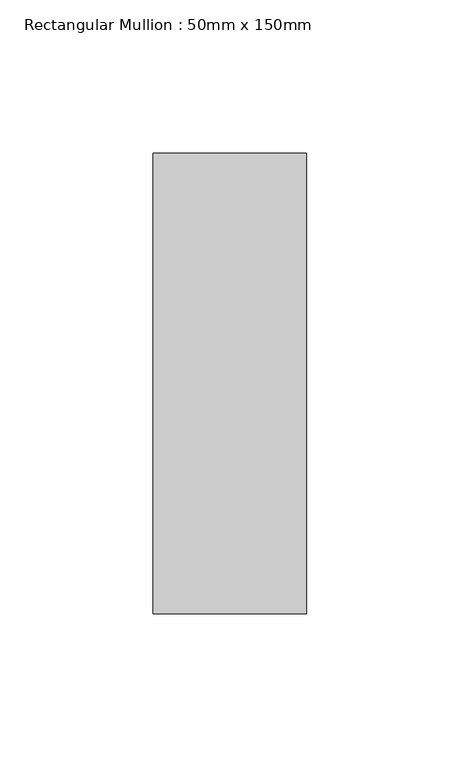
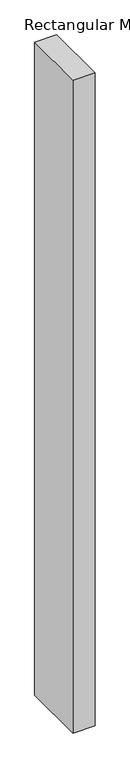
"""IFC4 building model written with IfcOpenShell, lengths in millimetres: member geometry, Rectangular Mullion : 50mm x 150mm."""

from ifc_helpers import new_model, si_unit, frame, origin, place, context, project, spatial, polyline, outline, extrude, source, transform, mapped, element, save


def rectangular_mullion_50mm_x_150mm_d9f1e9e9(model_context):
    return source(origin(), model_context, "Body", "SweptSolid", [
        extrude(outline(polyline([(0.0, 75.0), (0.0, -75.0), (-50.0, -75.0), (-50.0, 75.0), (0.0, 75.0)])), frame((0.0, 0.0, -1565.8160321), z_axis=(0.0, 0.0, 1.0), x_axis=(1.0, 0.0, 0.0)), (0.0, 0.0, 1.0), 1565.8160321),
    ])


if __name__ == "__main__":
    model = new_model("IFC4")
    model_context = context("Model", 3, world=origin())
    ifc_project = project(units=[si_unit("LENGTHUNIT", "METRE", prefix="MILLI")], contexts=[model_context])
    site = spatial("IfcSite", under=ifc_project)
    building = spatial("IfcBuilding", under=site)
    placement = place(None, origin())
    rectangular_mullion_50mm_x_150mm_shape = rectangular_mullion_50mm_x_150mm_d9f1e9e9(model_context)
    element("IfcMember", 1, ObjectType="Rectangular Mullion : 50mm x 150mm", at=placement, inside=building, context=model_context, shape_type="MappedRepresentation", body=[
        mapped(rectangular_mullion_50mm_x_150mm_shape, transform((0.0, 0.0, 0.0), x_axis=(1.0, 0.0, 0.0), y_axis=(0.0, 1.0, 0.0), z_axis=(0.0, 0.0, 1.0))),
    ])
    save(model, "model.ifc")

# Revit data of these elements
# Type "Rectangular Mullion : 50mm x 150mm"
#   built-in parameter 1007304 = 0.492126 (stored number, unit not read)
#   built-in parameter 1007301 = 0.082021 (stored number, unit not read)
#   built-in parameter 1007300 = 0.082021 (stored number, unit not read)
# Element 1 (IfcMember, "Rectangular Mullion : 50mm x 150mm")
#   Materials on its faces: "Aluminum"
# Materials
#   "Aluminum": class "Metal", colour RGB 244 244 244, transparency 0, Description = "Aluminum 6061", Cost = 0
